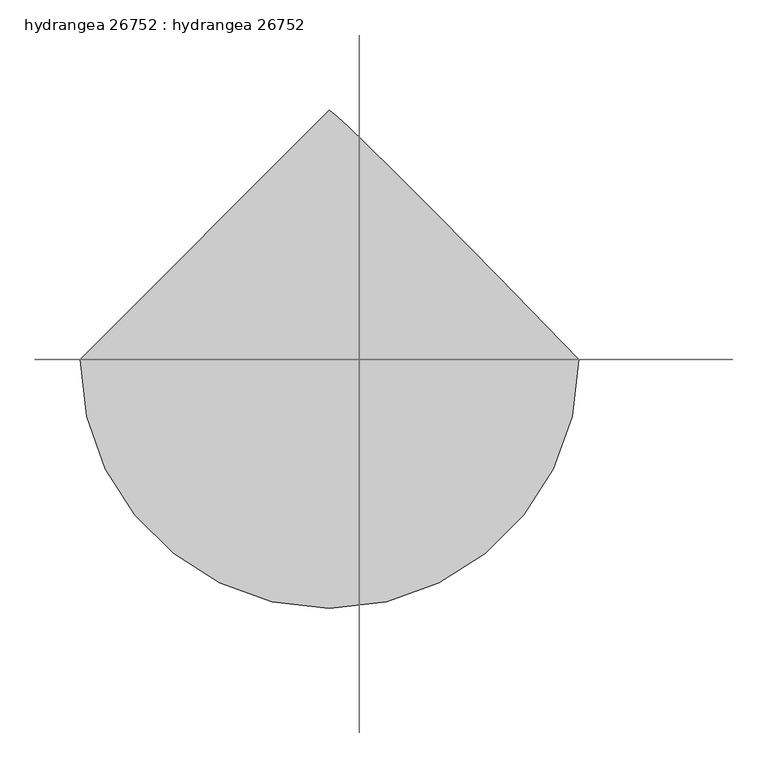
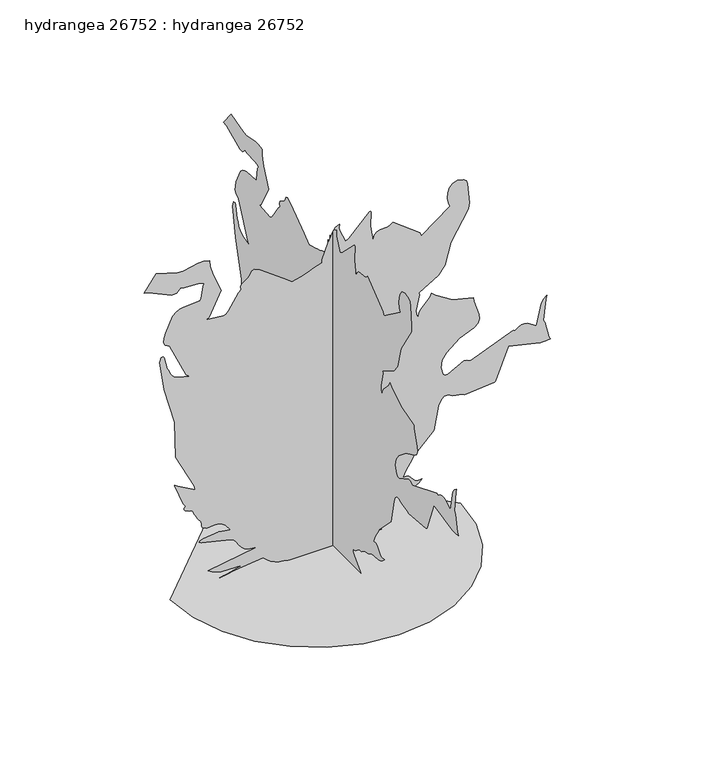
"""IFC4 building model written with IfcOpenShell, lengths in millimetres: proxy geometry, hydrangea 26752 : hydrangea 26752."""

import ifcopenshell
import ifcopenshell.guid

model = None  # the IFC model being written
_history = None  # IfcOwnerHistory: only IFC2X3 demands one
_inside = {}  # id of a spatial element -> (the spatial element, [elements in it])
_under = {}  # id of a project, library or spatial element -> (it, [spatial elements below it])
_declared = {}  # id of a project -> (the project, [libraries it declares])
_typed = {}  # id of a type object -> (the type object, [elements of that type])
_made_of = {}  # id of a material, layer set ... -> (it, [elements and type objects made of it])


def new_model(schema):
    """Start an empty IFC model of exactly this schema.

    Asked for "IFC4X3", IfcOpenShell would pick the latest addendum, in which some entities
    have other attributes; the version numbers below select the first issue.
    IFC2X3 requires an IfcOwnerHistory on every rooted entity: one is made here for all.
    """
    global model, _history
    if schema == "IFC4X3":
        model = ifcopenshell.file(schema_version=(4, 3, 0, 0))
    else:
        model = ifcopenshell.file(schema=schema)
    _inside.clear()
    _under.clear()
    _declared.clear()
    _typed.clear()
    _made_of.clear()
    _history = None
    if model.schema == "IFC2X3":
        org = make("IfcOrganization", Name="unknown")
        user = make(
            "IfcPersonAndOrganization",
            ThePerson=make("IfcPerson", FamilyName="unknown"),
            TheOrganization=org,
        )
        app = make(
            "IfcApplication",
            ApplicationDeveloper=org,
            Version="unknown",
            ApplicationFullName="unknown",
            ApplicationIdentifier="unknown",
        )
        _history = make(
            "IfcOwnerHistory",
            OwningUser=user,
            OwningApplication=app,
            ChangeAction="ADDED",
            CreationDate=0,
        )
    return model


def make(cls, **values):
    """One entity of the class cls with the attributes given. An attribute that is None is left unset."""
    return model.create_entity(
        cls, **{name: value for name, value in values.items() if value is not None}
    )


def rooted(cls, **values):
    """An entity with a GlobalId (a new one), such as an element, a storey or a relation."""
    return make(cls, GlobalId=ifcopenshell.guid.new(), OwnerHistory=_history, **values)


def si_unit(unit_type, name, prefix=None):
    """IfcSIUnit, for example si_unit("LENGTHUNIT", "METRE", prefix="MILLI")."""
    return make("IfcSIUnit", UnitType=unit_type, Prefix=prefix, Name=name)


def assignment(units):
    """IfcUnitAssignment: the units of a project."""
    return None if units is None else make("IfcUnitAssignment", Units=units)


def point(xyz):
    """IfcCartesianPoint."""
    return None if xyz is None else make("IfcCartesianPoint", Coordinates=xyz)


def direction(xyz):
    """IfcDirection."""
    return None if xyz is None else make("IfcDirection", DirectionRatios=xyz)


def frame(location, z_axis=None, x_axis=None):
    """IfcAxis2Placement3D, a coordinate frame: its origin and axes. An axis left out is left unset."""
    return make(
        "IfcAxis2Placement3D",
        Location=point(location),
        Axis=direction(z_axis),
        RefDirection=direction(x_axis),
    )


def origin():
    """The frame at (0, 0, 0) with its axes left unset."""
    return frame((0.0, 0.0, 0.0))


def place(relative_to, where):
    """IfcLocalPlacement: puts the frame where relative to a parent placement (None: the world)."""
    return make(
        "IfcLocalPlacement", PlacementRelTo=relative_to, RelativePlacement=where
    )


def context(
    kind, dimensions, precision=None, world=None, true_north=None, identifier=None
):
    """IfcGeometricRepresentationContext, for example the 3D "Model" context."""
    return make(
        "IfcGeometricRepresentationContext",
        ContextIdentifier=identifier,
        ContextType=kind,
        CoordinateSpaceDimension=dimensions,
        Precision=precision,
        WorldCoordinateSystem=world,
        TrueNorth=true_north,
    )


def project(units=None, contexts=None):
    """IfcProject with its units and contexts."""
    return rooted(
        "IfcProject",
        Name="project",
        RepresentationContexts=contexts,
        UnitsInContext=assignment(units),
    )


def spatial(cls, under=None, at=None, **own):
    """A site, building, storey or space (cls), placed at a placement, below another one or the project."""
    s = rooted(cls, ObjectPlacement=at, **own)
    if under is not None:
        _under.setdefault(under.id(), (under, []))[1].append(s)
    return s


def point_list(points):
    """IfcCartesianPointList2D or 3D."""
    cls = (
        "IfcCartesianPointList2D" if len(points[0]) == 2 else "IfcCartesianPointList3D"
    )
    return make(cls, CoordList=points)


def triangles(points, corners, closed=None, point_numbers=None):
    """IfcTriangulatedFaceSet: each triangle names its three corners, points numbered from 1."""
    return make(
        "IfcTriangulatedFaceSet",
        Coordinates=point_list(points),
        Closed=closed,
        CoordIndex=corners,
        PnIndex=point_numbers,
    )


def shape(context_of_items, identifier, shape_type, items):
    """IfcShapeRepresentation: the items that make up one representation, for example the "Body"."""
    return make(
        "IfcShapeRepresentation",
        ContextOfItems=context_of_items,
        RepresentationIdentifier=identifier,
        RepresentationType=shape_type,
        Items=items,
    )


def source(mapping_origin, context_of_items, identifier, shape_type, items):
    """IfcRepresentationMap: a shape defined once, which mapped items show again and again."""
    return make(
        "IfcRepresentationMap",
        MappingOrigin=mapping_origin,
        MappedRepresentation=shape(context_of_items, identifier, shape_type, items),
    )


def transform(
    local_origin,
    x_axis=None,
    y_axis=None,
    z_axis=None,
    scale=None,
    scale2=None,
    scale3=None,
    uniform=True,
):
    """IfcCartesianTransformationOperator3D, or its non-uniform kind. x_axis, y_axis, z_axis: its Axis1, 2, 3."""
    if uniform:
        return make(
            "IfcCartesianTransformationOperator3D",
            Axis1=direction(x_axis),
            Axis2=direction(y_axis),
            LocalOrigin=point(local_origin),
            Scale=scale,
            Axis3=direction(z_axis),
        )
    return make(
        "IfcCartesianTransformationOperator3DnonUniform",
        Axis1=direction(x_axis),
        Axis2=direction(y_axis),
        LocalOrigin=point(local_origin),
        Scale=scale,
        Axis3=direction(z_axis),
        Scale2=scale2,
        Scale3=scale3,
    )


def mapped(mapping_source, mapping_target):
    """IfcMappedItem: shows the shape of a source again, moved by a transform."""
    return make(
        "IfcMappedItem", MappingSource=mapping_source, MappingTarget=mapping_target
    )


def made_of(thing, what):
    """Note that an element or type object is made of a material, layer set ...; save() writes the relation."""
    if what is not None:
        _made_of.setdefault(what.id(), (what, []))[1].append(thing)
    return thing


def element(
    cls,
    number,
    at=None,
    inside=None,
    cuts=None,
    type_object=None,
    material=None,
    context=None,
    identifier="Body",
    shape_type=None,
    held_by="IfcProductDefinitionShape",
    body=None,
    shapes=None,
    **own,
):
    """One element of the class cls, such as IfcWall. Its Tag is "e" and its number.

    at: its placement. inside: the storey or other place that contains it. cuts: it is an
    opening in that element (IfcRelVoidsElement). A single representation is given by context,
    identifier, shape_type and body (its items); several are given by shapes. held_by: the class
    of the entity that holds the representations. save() writes the other relations.
    """
    e = rooted(cls, Tag="e%d" % number, ObjectPlacement=at, **own)
    if body is not None:
        shapes = [shape(context, identifier, shape_type, body)]
    if shapes is not None:
        e.Representation = make(held_by, Representations=shapes)
    if inside is not None:
        _inside.setdefault(inside.id(), (inside, []))[1].append(e)
    if cuts is not None:
        rooted(
            "IfcRelVoidsElement", RelatingBuildingElement=cuts, RelatedOpeningElement=e
        )
    if type_object is not None:
        _typed.setdefault(type_object.id(), (type_object, []))[1].append(e)
    return made_of(e, material)


def aggregate(whole, parts):
    """IfcRelAggregates: a whole, such as a stair, and the parts it consists of."""
    return rooted("IfcRelAggregates", RelatingObject=whole, RelatedObjects=parts)


def save(model, path):
    """Write the relations noted so far, then the file.

    IfcRelAggregates (storeys below a building ...), IfcRelContainedInSpatialStructure (elements
    in a storey), IfcRelDefinesByType, IfcRelAssociatesMaterial and IfcRelDeclares: one each for
    every whole, place, type object, material and project.
    """
    for whole, parts in _under.values():
        aggregate(whole, parts)
    for where, things in _inside.values():
        rooted(
            "IfcRelContainedInSpatialStructure",
            RelatedElements=things,
            RelatingStructure=where,
        )
    for kind, things in _typed.values():
        rooted("IfcRelDefinesByType", RelatedObjects=things, RelatingType=kind)
    for what, things in _made_of.values():
        rooted("IfcRelAssociatesMaterial", RelatedObjects=things, RelatingMaterial=what)
    for by, libraries in _declared.values():
        rooted("IfcRelDeclares", RelatingContext=by, RelatedDefinitions=libraries)
    model.write(path)


def hydrangea_26752_hydrangea_26752_6cd4de68(model_context):
    return source(origin(), model_context, "Body", "Tessellation", [
        triangles([(-464.7672343, 0.0, 3.02e-05), (-452.4787039, -106.4936905, 3.02e-05), (-417.4875984, -204.2914365, 3.02e-05), (-362.5905132, -290.5916013, 3.02e-05), (-290.5916013, -362.5905132, 3.02e-05), (-204.2911822, -417.4875984, 3.02e-05), (-106.4936905, -452.4787039, 3.02e-05), (2.03e-05, -464.7672343, 3.02e-05), (106.4939449, -452.4787039, 3.02e-05), (204.2914365, -417.4875984, 3.02e-05), (290.5916013, -362.5905132, 3.02e-05), (362.5905132, -290.5916013, 3.02e-05), (417.4875984, -204.2911822, 3.02e-05), (452.4787039, -106.4936905, 3.02e-05), (464.7672343, 4.06e-05, 3.02e-05), (313.7284884, 154.9290062, 3.02e-05), (201.7549816, 268.9964805, 3.02e-05), (122.337727, 349.0116546, 3.02e-05), (68.9646404, 401.7878663, 3.02e-05), (35.1246865, 434.1297149, 3.02e-05), (14.3067201, 452.8546257, 3.02e-05), (-6.09e-05, 464.7672343, 3.02e-05), (56.0289111, -377.7746518, 894.66276), (56.0289111, -434.8662978, 988.0256659), (56.0289111, -437.025323, 1007.8783058), (56.0289111, -431.6938534, 1074.0784075), (56.0289111, -427.5688871, 1084.5381615), (56.0289111, -420.2181004, 1091.4545998), (56.0289111, -399.2732306, 1096.0341894), (56.0289111, -384.089092, 1091.3859993), (56.0289111, -374.1170626, 1079.9991943), (56.0289111, -368.8109911, 1064.3553091), (56.0289111, -367.6197121, 1046.9435812), (56.0289111, -369.9971832, 1030.2455452), (56.0289111, -375.3946735, 1016.7479679), (56.0289111, -283.8809099, 949.5141357), (56.0289111, -278.4503729, 960.8348837), (56.0289111, -192.0161139, 1027.487138), (56.0289111, -183.512436, 1019.3997683), (56.0289111, -173.3158381, 1016.575304), (56.0289111, -151.4921339, 1016.077442), (56.0289111, -141.6905156, 1013.0776978), (56.0289111, -133.8441922, 1004.6956512), (56.0289111, -128.8665527, 988.2669302), (56.0289111, -120.2805761, 1038.0128763), (56.0289111, -121.9587531, 1087.6699471), (56.0289111, -121.3283319, 1088.8815737), (56.0289111, -120.3204537, 1089.2625824), (56.0289111, -119.0941387, 1088.975536), (56.0289111, -117.8101691, 1088.1856133), (56.0289111, -51.0174846, 1022.5290831), (56.0289111, -40.1538944, 1015.3484894), (56.0289111, -21.3923125, 1059.6105406), (56.0289111, -19.9031842, 1068.9729778), (56.0289111, -20.5441289, 1080.248089), (56.0289111, -9.1964113, 1074.4568727), (56.0289111, -0.5405762, 1063.7304199), (56.0289111, 13.2029357, 1031.7950146), (56.0289111, 15.0194446, 1031.1828426), (56.0289111, 16.1084712, 1040.5605406), (56.0289111, 15.8290449, 1030.10333), (56.0289111, 34.9326629, 980.1719301), (56.0289111, 34.6535171, 969.7147923), (56.0289111, 46.9016657, 965.6583538), (56.0289111, 59.853396, 960.979715), (56.0289111, 73.3885619, 956.0013124), (56.0289111, 87.3888065, 951.0482718), (56.0289111, 101.7342336, 946.4457911), (56.0289111, 116.3062366, 942.5138363), (56.0289111, 130.9854187, 939.5776056), (56.0289111, 158.8299491, 961.2921232), (56.0289111, 234.3038488, 1015.5618484), (56.0289111, 252.5433605, 1023.7431805), (56.0289111, 260.6957517, 1020.4259411), (56.0289111, 264.4829115, 1008.7952557), (56.0289111, 270.9573709, 1001.4368385), (56.0289111, 292.1841821, 987.7081707), (56.0289111, 295.084859, 980.1414814), (56.0289111, 293.5100641, 968.1907574), (56.0289111, 301.5567932, 960.9593674), (56.0289111, 333.5786213, 911.8103325), (56.0289111, 341.9555446, 903.575588), (56.0289111, 350.6474195, 900.6063652), (56.0289111, 405.2778059, 906.5576008), (56.0289111, 397.091387, 912.3182957), (56.0289111, 357.3022459, 989.5521715), (56.0289111, 383.3829941, 1051.2462982), (56.0289111, 392.869915, 1083.2706516), (56.0289111, 394.0713315, 1102.6610378), (56.0289111, 413.8020676, 1107.4693199), (56.0289111, 431.2518745, 1106.8977705), (56.0289111, 479.0928497, 1096.097703), (56.0289111, 496.5959965, 1097.2025774), (56.0289111, 565.8923844, 1117.6013323), (56.0289111, 605.1150993, 1065.3077946), (56.0289111, 590.4389603, 1063.2046526), (56.0289111, 515.963528, 1028.2542423), (56.0289111, 499.8980115, 1030.0398165), (56.0289111, 487.4520052, 1042.8973166), (56.0289111, 476.9008324, 1039.305748), (56.0289111, 431.2823596, 1037.8351255), (56.0289111, 421.2823886, 1035.6633831), (56.0289111, 412.7479531, 1030.7561245), (56.0289111, 416.4106656, 1023.8879391), (56.0289111, 422.1561361, 984.398489), (56.0289111, 425.8213557, 977.5278328), (56.0289111, 478.1860737, 974.7465345), (56.0289111, 490.5939646, 971.7493338), (56.0289111, 502.2144762, 965.7473019), (56.0289111, 512.7834532, 955.7015488), (56.0289111, 536.4029417, 906.3493286), (56.0289111, 540.7590348, 890.4260273), (56.0289111, 541.4473649, 876.4001392), (56.0289111, 536.9465132, 865.9378418), (56.0289111, 523.4413055, 857.3729576), (56.0289111, 470.3247439, 742.9737631), (56.0289111, 459.1462111, 734.3275612), (56.0289111, 495.4784048, 743.0092987), (56.0289111, 506.2683349, 747.8099504), (56.0289111, 515.3336246, 754.7263887), (56.0289111, 522.0366674, 764.454574), (56.0289111, 525.7400024, 777.6930828), (56.0289111, 531.1476665, 784.7339321), (56.0289111, 539.8243172, 825.0565435), (56.0289111, 543.8298866, 829.879941), (56.0289111, 550.6015663, 829.2856459), (56.0289111, 555.6434461, 813.3064613), (56.0289111, 540.8123746, 716.5628025), (56.0289111, 507.4392663, 594.6655191), (56.0289111, 503.093347, 475.8365441), (56.0289111, 444.0484045, 359.0446904), (56.0289111, 441.1045435, 344.0002235), (56.0289111, 497.2995872, 374.7622267), (56.0289111, 506.1286268, 381.752316), (56.0289111, 507.3122755, 379.8777938), (56.0289111, 479.3442879, 309.3622215), (56.0289111, 471.5769931, 298.1760402), (56.0289111, 476.8474926, 293.4109968), (56.0289111, 476.8347754, 288.7729441), (56.0289111, 473.0577893, 284.5159002), (56.0289111, 460.289201, 278.1963731), (56.0289111, 454.3303714, 276.6495199), (56.0289111, 450.6829196, 276.5250544), (56.0289111, 447.9727289, 270.8405358), (56.0289111, 445.4428688, 265.374445), (56.0289111, 442.9105016, 259.9769365), (56.0289111, 440.1901734, 254.4981467), (56.0289111, 437.1015175, 248.789756), (56.0289111, 433.4642395, 242.6990667), (56.0289111, 429.0903422, 236.0780501), (56.0289111, 423.9341526, 231.4173971), (56.0289111, 421.2519035, 226.5421133), (56.0289111, 420.2282742, 221.6594716), (56.0289111, 420.0530305, 216.9764544), (56.0289111, 419.910779, 212.7001166), (56.0289111, 418.9912857, 209.0374223), (56.0289111, 416.4817732, 206.1956808), (56.0289111, 404.3481751, 201.1304013), (56.0289111, 392.979138, 200.8065475), (56.0289111, 381.7802576, 202.325223), (56.0289111, 370.1622894, 202.7872406), (56.0289111, 357.5257424, 199.293722), (56.0289111, 343.2814084, 188.9454982), (56.0289111, 326.8374267, 168.843146), (56.0289111, 363.7335394, 174.8182537), (56.0289111, 415.2447847, 168.959745), (56.0289111, 424.7621907, 165.1799612), (56.0289111, 427.6882476, 161.3724901), (56.0289111, 422.6031655, 158.3819023), (56.0289111, 326.8374267, 135.2257031), (56.0289111, 316.3675352, 128.5444794), (56.0289111, 308.4071926, 119.1548454), (56.0289111, 301.2011826, 108.4708318), (56.0289111, 292.9842786, 97.9059425), (56.0289111, 281.9936886, 88.8741991), (56.0289111, 266.4742689, 82.7891145), (56.0289111, 244.6604659, 81.0642016), (56.0289111, 399.6745505, 54.9174055), (56.0289111, 387.1320385, 46.4490362), (56.0289111, 358.6535079, 37.4287247), (56.0289111, 291.3510571, 36.2410178), (56.0289111, 337.9144032, 23.9287606), (56.0289111, 349.4180614, 21.3156048), (56.0289111, 362.3212709, 18.4984871), (56.0289111, 355.630909, 19.454849), (56.0289111, 338.5316257, 22.4599004), (56.0289111, 314.6454383, 26.6484415), (56.0289111, 223.7308386, 37.9362155), (56.0289111, 211.5466986, 26.1533955), (56.0289111, 198.7755668, 17.3074794), (56.0289111, 185.515475, 10.9090339), (56.0289111, 171.8642371, 6.4684733), (56.0289111, 157.9193579, 3.4965937), (56.0289111, 143.7791599, 1.5035523), (56.0289111, 129.5409211, 0.0), (56.0289111, -156.3006158, 8.5e-06), (56.0289111, -151.6640893, 6.8894283), (56.0289111, -116.3057279, 38.9204668), (56.0289111, -111.4957199, 47.331436), (56.0289111, -111.590972, 55.6176853), (56.0289111, -119.3379828, 56.8782915), (56.0289111, -125.2241879, 59.5351333), (56.0289111, -130.2038621, 63.1188217), (56.0289111, -135.2315439, 67.1597133), (56.0289111, -141.2622714, 71.1881602), (56.0289111, -149.2498198, 74.7345099), (56.0289111, -160.1494906, 77.329128), (56.0289111, -168.9650681, 83.9521794), (56.0289111, -176.5355544, 87.5539036), (56.0289111, -196.7577757, 92.3169214), (56.0289111, -204.3280077, 95.9186456), (56.0289111, -213.1436033, 102.5419604), (56.0289111, -254.4092531, 106.5686224), (56.0289111, -265.3388912, 110.053257), (56.0289111, -275.7884532, 116.2788036), (56.0289111, -285.3972962, 126.1210626), (56.0289111, -270.7287694, 125.7187253), (56.0289111, -261.0386631, 129.5500684), (56.0289111, -244.0602664, 149.2523633), (56.0289111, -236.5088377, 152.8248832), (56.0289111, -225.0498715, 152.0344246), (56.0289111, -234.5898597, 172.6625532), (56.0289111, -246.2180017, 193.2690897), (56.0289111, -259.5756166, 213.3033683), (56.0289111, -323.1010995, 276.6977727), (56.0289111, -338.0566183, 354.6326777), (56.0289111, -345.6055398, 371.0131823), (56.0289111, -356.2354506, 380.7922002), (56.0289111, -370.7261358, 381.2874825), (56.0289111, -376.1719153, 376.5935466), (56.0289111, -382.951189, 373.9163844), (56.0289111, -414.431971, 368.0820022), (56.0289111, -421.1503109, 364.0103757), (56.0289111, -516.6848866, 372.087608), (56.0289111, -521.0689213, 374.2821688), (56.0289111, -561.6327971, 477.6729873), (56.0289111, -663.3141632, 454.759633), (56.0289111, -683.0017696, 454.2617709), (56.0289111, -696.6263014, 456.4588752), (56.0289111, -691.4650612, 464.9628256), (56.0289111, -679.3771362, 518.9251568), (56.0289111, -674.215896, 527.4291072), (56.0289111, -681.6479279, 594.9220805), (56.0289111, -685.4224068, 606.8042041), (56.0289111, -674.9575659, 597.7338638), (56.0289111, -667.4314991, 587.1039531), (56.0289111, -651.805418, 516.2225965), (56.0289111, -623.5224787, 533.9975653), (56.0289111, -613.96703, 536.3114865), (56.0289111, -604.0863831, 535.7831758), (56.0289111, -593.7181206, 531.7852003), (56.0289111, -582.7021142, 523.6927437), (56.0289111, -577.4646432, 527.2970295), (56.0289111, -440.4085831, 471.9960809), (56.0289111, -429.7609045, 477.805065), (56.0289111, -420.0225454, 479.0471403), (56.0289111, -367.9321567, 451.6074635), (56.0289111, -358.5290606, 450.3882792), (56.0289111, -353.3322121, 456.9262522), (56.0289111, -345.7960078, 481.3356634), (56.0289111, -350.0683125, 504.1753667), (56.0289111, -363.3880663, 525.0059266), (56.0289111, -406.1337856, 558.9200629), (56.0289111, -451.9579871, 579.6160017), (56.0289111, -465.1685543, 589.0190978), (56.0289111, -469.6389573, 603.0043633), (56.0289111, -467.9142806, 619.826774), (56.0289111, -451.0918336, 669.8597666), (56.0289111, -450.0987256, 680.5760456), (56.0289111, -383.0096157, 698.4017744), (56.0289111, -329.3240845, 731.7240864), (56.0289111, -316.5631265, 743.6087534), (56.0289111, -311.5136164, 731.6199503), (56.0289111, -280.6932047, 700.0375757), (56.0289111, -275.2499687, 690.0807707), (56.0289111, -272.6744173, 676.8397184), (56.0289111, -266.9721128, 689.0418806), (56.0289111, -265.8748323, 702.5623489), (56.0289111, -277.0838502, 752.2879475), (56.0289111, -276.1770741, 759.2500952), (56.0289111, -338.0413939, 796.367161), (56.0289111, -358.8363819, 823.4360029), (433.8020459, 5.25e-05, 894.66276), (490.8936919, 6.21e-05, 988.0256659), (493.0552242, 6.39e-05, 1007.8783058), (487.7237909, 6.93e-05, 1074.0784075), (483.5988247, 7.01e-05, 1084.5381615), (476.2454945, 7.04e-05, 1091.4545998), (455.3006247, 7.02e-05, 1096.0341894), (440.1164861, 6.93e-05, 1091.3859993), (430.1470001, 6.81e-05, 1079.9991943), (424.8383852, 6.66e-05, 1064.3553091), (423.6496496, 6.51e-05, 1046.9435812), (426.0270844, 6.37e-05, 1030.2455452), (431.4246111, 6.27e-05, 1016.7479679), (339.9082858, 5.44e-05, 949.5141357), (334.477767, 5.52e-05, 960.8348837), (248.0447615, 5.82e-05, 1027.487138), (239.541338, 5.73e-05, 1019.3997683), (229.3447583, 5.67e-05, 1016.575304), (207.5210541, 5.6e-05, 1016.077442), (197.7191814, 5.55e-05, 1013.0776978), (189.8731124, 5.45e-05, 1004.6956512), (184.8952004, 5.3e-05, 988.2669302), (176.3092419, 5.66e-05, 1038.0128763), (177.9874098, 6.11e-05, 1087.6699471), (177.3572339, 6.11e-05, 1088.8815737), (176.3491196, 6.1e-05, 1089.2625824), (175.1227954, 6.09e-05, 1088.975536), (173.8390802, 6.07e-05, 1088.1856133), (107.0464002, 5.35e-05, 1022.5290831), (96.182801, 5.27e-05, 1015.3484894), (77.4210737, 5.59e-05, 1059.6105406), (75.9321248, 5.66e-05, 1068.9729778), (76.5729696, 5.75e-05, 1080.248089), (65.2252475, 5.67e-05, 1074.4568727), (56.5694259, 5.55e-05, 1063.7304199), (42.8259742, 5.23e-05, 1031.7950146), (41.0093655, 5.23e-05, 1031.1828426), (39.9204648, 5.31e-05, 1040.5605406), (40.1998673, 5.22e-05, 1030.10333), (21.0960983, 4.75e-05, 980.1719301), (21.3753963, 4.66e-05, 969.7147923), (9.1270438, 4.59e-05, 965.6583538), (-3.8244574, 4.51e-05, 960.979715), (-17.3597019, 4.43e-05, 956.0013124), (-31.3598954, 4.34e-05, 951.0482718), (-45.7053225, 4.26e-05, 946.4457911), (-60.2773209, 4.18e-05, 942.5138363), (-74.9565076, 4.11e-05, 939.5776056), (-102.801038, 4.21e-05, 961.2921232), (-178.2749468, 4.45e-05, 1015.5618484), (-196.5144585, 4.46e-05, 1023.7431805), (-204.6668497, 4.41e-05, 1020.4259411), (-208.4534826, 4.3e-05, 1008.7952557), (-214.9284508, 4.22e-05, 1001.4368385), (-236.1547533, 4.05e-05, 987.7081707), (-239.055957, 3.97e-05, 980.1414814), (-237.481907, 3.88e-05, 968.1907574), (-245.5273643, 3.79e-05, 960.9593674), (-277.5486837, 3.28e-05, 911.8103325), (-285.9281505, 3.19e-05, 903.575588), (-294.6200436, 3.14e-05, 900.6063652), (-349.2479047, 3.02e-05, 906.5576008), (-341.0639929, 3.09e-05, 912.3182957), (-301.2723083, 3.86e-05, 989.5521715), (-327.3530565, 4.31e-05, 1051.2462982), (-336.8399775, 4.55e-05, 1083.2706516), (-338.0413939, 4.71e-05, 1102.6610378), (-357.77213, 4.69e-05, 1107.4693199), (-375.2244804, 4.63e-05, 1106.8977705), (-423.0654556, 4.4e-05, 1096.097703), (-440.5660953, 4.36e-05, 1097.2025774), (-509.8649903, 4.32e-05, 1117.6013323), (-549.0851618, 3.76e-05, 1065.3077946), (-534.4115662, 3.79e-05, 1063.2046526), (-459.9361339, 3.72e-05, 1028.2542423), (-443.8706174, 3.78e-05, 1030.0398165), (-431.4246111, 3.93e-05, 1042.8973166), (-420.8734383, 3.93e-05, 1039.305748), (-375.252422, 4.05e-05, 1037.8351255), (-365.252451, 4.06e-05, 1035.6633831), (-356.7180519, 4.05e-05, 1030.7561245), (-360.3832715, 3.98e-05, 1023.8879391), (-366.128742, 3.63e-05, 984.398489), (-369.7914182, 3.56e-05, 977.5278328), (-422.1586796, 3.38e-05, 974.7465345), (-434.5666068, 3.32e-05, 971.7493338), (-446.184575, 3.23e-05, 965.7473019), (-456.7535156, 3.12e-05, 955.7015488), (-480.3730042, 2.63e-05, 906.3493286), (-484.7290973, 2.48e-05, 890.4260273), (-485.4174637, 2.36e-05, 876.4001392), (-480.9165756, 2.29e-05, 865.9378418), (-467.4139114, 2.25e-05, 857.3729576), (-414.2948427, 1.45e-05, 742.9737631), (-403.118817, 1.41e-05, 734.3275612), (-439.4484673, 1.37e-05, 743.0092987), (-450.2383973, 1.38e-05, 747.8099504), (-459.303687, 1.42e-05, 754.7263887), (-466.0067662, 1.48e-05, 764.454574), (-469.7100649, 1.58e-05, 777.6930828), (-475.117729, 1.62e-05, 784.7339321), (-483.7943796, 1.93e-05, 825.0565435), (-487.7999854, 1.96e-05, 829.879941), (-494.5741722, 1.93e-05, 829.2856459), (-499.6160883, 1.78e-05, 813.3064613), (-484.782437, 1.01e-05, 716.5628025), (-451.4119085, 9e-07, 594.6655191), (-447.0659529, -9e-06, 475.8365441), (-388.0210467, -1.71e-05, 359.0446904), (-385.0746423, -1.83e-05, 344.0002235), (-441.2721931, -1.73e-05, 374.7622267), (-450.1012327, -1.7e-05, 381.752316), (-451.2848814, -1.73e-05, 379.8777938), (-423.3143867, -2.24e-05, 309.3622215), (-415.549599, -2.3e-05, 298.1760402), (-420.817555, -2.36e-05, 293.4109968), (-420.8048378, -2.39e-05, 288.7729441), (-417.0303952, -2.41e-05, 284.5159002), (-404.2592634, -2.42e-05, 278.1963731), (-398.3029773, -2.42e-05, 276.6495199), (-394.6555255, -2.42e-05, 276.5250544), (-391.9453348, -2.46e-05, 270.8405358), (-389.4129676, -2.5e-05, 265.374445), (-386.880564, -2.54e-05, 259.9769365), (-384.1602359, -2.58e-05, 254.4981467), (-381.0741234, -2.62e-05, 248.789756), (-377.4343019, -2.65e-05, 242.6990667), (-373.0604047, -2.7e-05, 236.0780501), (-367.9067585, -2.72e-05, 231.4173971), (-365.221966, -2.76e-05, 226.5421133), (-364.1983366, -2.8e-05, 221.6594716), (-364.0230929, -2.84e-05, 216.9764544), (-363.8808414, -2.87e-05, 212.7001166), (-362.9613482, -2.9e-05, 209.0374223), (-360.4543791, -2.92e-05, 206.1956808), (-348.320781, -2.92e-05, 201.1304013), (-336.9492004, -2.89e-05, 200.8065475), (-325.7528635, -2.84e-05, 202.325223), (-314.1323519, -2.81e-05, 202.7872406), (-301.4983665, -2.8e-05, 199.293722), (-287.2540325, -2.84e-05, 188.9454982), (-270.8075073, -2.96e-05, 168.843146), (-307.7036018, -3e-05, 174.8182537), (-359.2173906, -3.17e-05, 168.959745), (-368.7322532, -3.24e-05, 165.1799612), (-371.6583464, -3.32e-05, 161.3724901), (-366.5732643, -3.31e-05, 158.3819023), (-270.8075073, -3.24e-05, 135.2257031), (-260.3376158, -3.27e-05, 128.5444794), (-252.3792717, -3.32e-05, 119.1548454), (-245.1717719, -3.39e-05, 108.4708318), (-236.9543411, -3.46e-05, 97.9059425), (-225.9652771, -3.51e-05, 88.8741991), (-210.44484, -3.51e-05, 82.7891145), (-188.6315457, -3.46e-05, 81.0642016), (-343.6446493, -4.14e-05, 54.9174055), (-331.1021009, -4.15e-05, 46.4490362), (-302.6235885, -4.14e-05, 37.4287247), (-235.3221369, -3.98e-05, 36.2410178), (-281.887009, -4.21e-05, 23.9287856), (-293.3906855, -4.27e-05, 21.3156298), (-306.2913697, -4.33e-05, 18.498512), (-299.6009896, -4.31e-05, 19.454874), (-282.5016881, -4.23e-05, 22.4599277), (-258.6180442, -4.13e-05, 26.6484415), (-167.7021728, -3.76e-05, 37.9362155), (-155.5177784, -3.82e-05, 26.1533955), (-142.7466466, -3.86e-05, 17.3074794), (-129.4865639, -3.88e-05, 10.9090589), (-115.8353169, -3.87e-05, 6.4684733), (-101.8904468, -3.85e-05, 3.496619), (-87.7502488, -3.83e-05, 1.5035625), (-73.5122598, -3.8e-05, 9.2e-06), (212.3292817, -2.95e-05, 5.3e-06), (207.6930094, -2.9e-05, 6.8894283), (172.3346299, -2.74e-05, 38.9204668), (167.52464, -2.68e-05, 47.331436), (167.6196379, -2.61e-05, 55.6176853), (175.3668939, -2.58e-05, 56.8782915), (181.2528355, -2.54e-05, 59.5351333), (186.2325279, -2.49e-05, 63.1188217), (191.2602007, -2.44e-05, 67.1597133), (197.2911916, -2.39e-05, 71.1881602), (205.2787309, -2.34e-05, 74.7345099), (216.1781383, -2.29e-05, 77.329128), (224.9937339, -2.2e-05, 83.9521794), (232.5642021, -2.15e-05, 87.5539036), (252.7864416, -2.05e-05, 92.3169214), (260.3579453, -2e-05, 95.9186456), (269.1717423, -1.91e-05, 102.5419604), (310.4366472, -1.75e-05, 106.5686224), (321.3688288, -1.69e-05, 110.0530027), (331.8183726, -1.61e-05, 116.2788036), (341.4272338, -1.5e-05, 126.1210626), (326.7586887, -1.55e-05, 125.7187253), (317.0660391, -1.54e-05, 129.5500684), (300.0886597, -1.43e-05, 149.2523633), (292.5372311, -1.42e-05, 152.8248832), (281.0792822, -1.46e-05, 152.0344246), (290.6195429, -1.26e-05, 172.6625532), (302.2476667, -1.05e-05, 193.2690897), (315.6030107, -8.4e-06, 213.3033683), (379.1284936, -1.2e-06, 276.6977727), (394.0840124, 5.8e-06, 354.6326777), (401.6328976, 7.5e-06, 371.0131823), (412.2628083, 8.6e-06, 380.7922002), (426.7535299, 9.1e-06, 381.2874825), (432.1993094, 8.8e-06, 376.5935466), (438.9785831, 8.8e-06, 373.9163844), (470.4619085, 9.3e-06, 368.0820022), (477.1802121, 9.1e-06, 364.0103757), (572.7148241, 1.25e-05, 372.087608), (577.0988588, 1.3e-05, 374.2821688), (617.6601912, 2.29e-05, 477.6729873), (719.3415573, 2.4e-05, 454.759633), (739.0291637, 2.45e-05, 454.2617709), (752.6562389, 2.51e-05, 456.4588752), (747.4949987, 2.57e-05, 464.9628256), (735.4070738, 2.99e-05, 518.9251568), (730.2458336, 3.04e-05, 527.4291072), (737.6778654, 3.63e-05, 594.9220805), (741.4498009, 3.74e-05, 606.8042041), (730.9875034, 3.64e-05, 597.7338638), (723.4614367, 3.53e-05, 587.1039531), (707.8328121, 2.88e-05, 516.2225965), (679.5498728, 2.95e-05, 533.9975653), (669.9969675, 2.94e-05, 536.3114865), (660.1163206, 2.91e-05, 535.7831758), (649.7455147, 2.84e-05, 531.7852003), (638.729472, 2.74e-05, 523.6927437), (633.492001, 2.76e-05, 527.2970295), (496.4359772, 1.88e-05, 471.9960809), (485.7882986, 1.9e-05, 477.805065), (476.0524467, 1.88e-05, 479.0471403), (423.9620942, 1.49e-05, 451.6074635), (414.5564547, 1.45e-05, 450.3882792), (409.3621496, 1.49e-05, 456.9262522), (401.8259454, 1.72e-05, 481.3356634), (406.09825, 1.94e-05, 504.1753667), (419.4180038, 2.15e-05, 525.0059266), (462.1637232, 2.53e-05, 558.9200629), (507.9853812, 2.82e-05, 579.6160017), (521.1984919, 2.94e-05, 589.0190978), (525.6663514, 3.07e-05, 603.0043633), (523.9442182, 3.21e-05, 619.826774), (507.1192277, 3.58e-05, 669.8597666), (506.1286268, 3.66e-05, 680.5760456), (439.0370098, 3.62e-05, 698.4017744), (385.3514786, 3.74e-05, 731.7240864), (372.593064, 3.8e-05, 743.6087534), (367.5409741, 3.68e-05, 731.6199503), (336.7231241, 3.32e-05, 700.0375757), (331.2773809, 3.22e-05, 690.0807707), (328.7043549, 3.11e-05, 676.8397184), (323.0020503, 3.19e-05, 689.0418806), (321.9022264, 3.3e-05, 702.5623489), (333.1112443, 3.76e-05, 752.2879475), (332.2044683, 3.81e-05, 759.2500952), (394.0713315, 4.31e-05, 796.367161), (414.8663195, 4.6e-05, 823.4360029)], [[21, 22, 1], [20, 21, 1], [19, 20, 1], [18, 19, 1], [17, 18, 1], [17, 1, 2], [17, 2, 3], [17, 3, 4], [16, 17, 4], [16, 4, 5], [16, 5, 6], [16, 6, 7], [16, 7, 8], [16, 8, 9], [16, 9, 10], [16, 10, 11], [16, 11, 12], [15, 16, 12], [14, 15, 12], [13, 14, 12], [183, 184, 185], [59, 60, 61], [183, 185, 186], [182, 183, 186], [243, 244, 245], [177, 178, 179], [215, 216, 217], [195, 196, 197], [195, 197, 198], [182, 186, 187], [181, 182, 187], [181, 187, 188], [54, 55, 56], [94, 95, 96], [238, 239, 240], [195, 198, 199], [271, 272, 273], [167, 168, 169], [133, 134, 135], [214, 215, 217], [214, 217, 218], [177, 179, 180], [177, 180, 181], [166, 167, 169], [165, 166, 169], [164, 165, 169], [164, 169, 170], [37, 38, 39], [213, 214, 218], [94, 96, 97], [93, 94, 97], [93, 97, 98], [93, 98, 99], [92, 93, 99], [92, 99, 100], [92, 100, 101], [91, 92, 101], [90, 91, 101], [90, 101, 102], [89, 90, 102], [88, 89, 102], [87, 88, 102], [87, 102, 103], [195, 199, 200], [54, 56, 57], [53, 54, 57], [243, 245, 246], [242, 243, 246], [242, 246, 247], [241, 242, 247], [268, 269, 270], [87, 103, 104], [86, 87, 104], [86, 104, 105], [86, 105, 106], [85, 86, 106], [84, 85, 106], [133, 135, 136], [132, 133, 136], [132, 136, 137], [53, 57, 58], [125, 126, 127], [124, 125, 127], [123, 124, 127], [123, 127, 128], [122, 123, 128], [121, 122, 128], [120, 121, 128], [119, 120, 128], [52, 53, 58], [177, 181, 188], [118, 119, 128], [213, 218, 219], [213, 219, 220], [213, 220, 221], [212, 213, 221], [117, 118, 128], [164, 170, 171], [237, 238, 240], [237, 240, 241], [237, 241, 247], [237, 247, 248], [237, 248, 249], [237, 249, 250], [237, 250, 251], [237, 251, 252], [236, 237, 252], [236, 252, 253], [236, 253, 254], [235, 236, 254], [234, 235, 254], [233, 234, 254], [232, 233, 254], [232, 254, 255], [232, 255, 256], [232, 256, 257], [231, 232, 257], [230, 231, 257], [229, 230, 257], [229, 257, 258], [228, 229, 258], [84, 106, 107], [84, 107, 108], [84, 108, 109], [84, 109, 110], [84, 110, 111], [84, 111, 112], [84, 112, 113], [84, 113, 114], [84, 114, 115], [84, 115, 116], [84, 116, 117], [83, 84, 117], [270, 271, 273], [73, 74, 75], [72, 73, 75], [137, 138, 139], [137, 139, 140], [137, 140, 141], [132, 137, 141], [132, 141, 142], [132, 142, 143], [72, 75, 76], [227, 228, 258], [227, 258, 259], [117, 128, 129], [224, 225, 226], [46, 47, 48], [46, 48, 49], [46, 49, 50], [45, 46, 50], [45, 50, 51], [44, 45, 51], [44, 51, 52], [211, 212, 221], [210, 211, 221], [209, 210, 221], [82, 83, 117], [270, 273, 274], [270, 274, 275], [270, 275, 276], [264, 265, 266], [264, 266, 267], [264, 267, 268], [264, 268, 270], [263, 264, 270], [263, 270, 276], [262, 263, 276], [261, 262, 276], [52, 58, 59], [52, 59, 61], [52, 61, 62], [52, 62, 63], [44, 52, 63], [260, 261, 276], [71, 72, 76], [71, 76, 77], [71, 77, 78], [71, 78, 79], [71, 79, 80], [70, 71, 80], [70, 80, 81], [70, 81, 82], [70, 82, 117], [70, 117, 129], [70, 129, 130], [70, 130, 131], [69, 70, 131], [68, 69, 131], [67, 68, 131], [67, 131, 132], [66, 67, 132], [65, 66, 132], [64, 65, 132], [63, 64, 132], [44, 63, 132], [132, 143, 144], [44, 132, 144], [44, 144, 145], [44, 145, 146], [44, 146, 147], [44, 147, 148], [44, 148, 149], [44, 149, 150], [44, 150, 151], [44, 151, 152], [44, 152, 153], [44, 153, 154], [44, 154, 155], [44, 155, 156], [44, 156, 157], [44, 157, 158], [44, 158, 159], [44, 159, 160], [44, 160, 161], [44, 161, 162], [44, 162, 163], [44, 163, 164], [44, 164, 171], [44, 171, 172], [44, 172, 173], [44, 173, 174], [44, 174, 175], [44, 175, 176], [44, 176, 177], [44, 177, 188], [44, 188, 189], [44, 189, 190], [44, 190, 191], [44, 191, 192], [44, 192, 193], [44, 193, 194], [44, 194, 195], [44, 195, 200], [44, 200, 201], [44, 201, 202], [44, 202, 203], [44, 203, 204], [44, 204, 205], [44, 205, 206], [44, 206, 207], [44, 207, 208], [44, 208, 209], [44, 209, 221], [44, 221, 222], [44, 222, 223], [44, 223, 224], [44, 224, 226], [44, 226, 227], [44, 227, 259], [44, 259, 260], [43, 44, 260], [42, 43, 260], [29, 30, 31], [28, 29, 31], [28, 31, 32], [27, 28, 32], [26, 27, 32], [26, 32, 33], [26, 33, 34], [26, 34, 35], [25, 26, 35], [24, 25, 35], [23, 24, 35], [23, 35, 36], [282, 23, 36], [281, 282, 36], [280, 281, 36], [37, 39, 40], [280, 36, 37], [280, 37, 40], [280, 40, 41], [280, 41, 42], [279, 280, 42], [278, 279, 42], [277, 278, 42], [277, 42, 260], [277, 260, 276], [443, 444, 445], [319, 320, 321], [443, 445, 446], [442, 443, 446], [503, 504, 505], [437, 438, 439], [475, 476, 477], [455, 456, 457], [455, 457, 458], [442, 446, 447], [441, 442, 447], [441, 447, 448], [314, 315, 316], [354, 355, 356], [498, 499, 500], [455, 458, 459], [531, 532, 533], [427, 428, 429], [393, 394, 395], [474, 475, 477], [474, 477, 478], [437, 439, 440], [437, 440, 441], [426, 427, 429], [425, 426, 429], [424, 425, 429], [424, 429, 430], [297, 298, 299], [473, 474, 478], [354, 356, 357], [353, 354, 357], [353, 357, 358], [353, 358, 359], [352, 353, 359], [352, 359, 360], [352, 360, 361], [351, 352, 361], [350, 351, 361], [350, 361, 362], [349, 350, 362], [348, 349, 362], [347, 348, 362], [347, 362, 363], [455, 459, 460], [314, 316, 317], [313, 314, 317], [503, 505, 506], [502, 503, 506], [502, 506, 507], [501, 502, 507], [528, 529, 530], [347, 363, 364], [346, 347, 364], [346, 364, 365], [346, 365, 366], [345, 346, 366], [344, 345, 366], [393, 395, 396], [392, 393, 396], [392, 396, 397], [313, 317, 318], [385, 386, 387], [384, 385, 387], [383, 384, 387], [383, 387, 388], [382, 383, 388], [381, 382, 388], [380, 381, 388], [379, 380, 388], [312, 313, 318], [437, 441, 448], [378, 379, 388], [473, 478, 479], [473, 479, 480], [473, 480, 481], [472, 473, 481], [377, 378, 388], [424, 430, 431], [497, 498, 500], [497, 500, 501], [497, 501, 507], [497, 507, 508], [497, 508, 509], [497, 509, 510], [497, 510, 511], [497, 511, 512], [496, 497, 512], [496, 512, 513], [496, 513, 514], [495, 496, 514], [494, 495, 514], [493, 494, 514], [492, 493, 514], [492, 514, 515], [492, 515, 516], [492, 516, 517], [491, 492, 517], [490, 491, 517], [489, 490, 517], [489, 517, 518], [488, 489, 518], [344, 366, 367], [344, 367, 368], [344, 368, 369], [344, 369, 370], [344, 370, 371], [344, 371, 372], [344, 372, 373], [344, 373, 374], [344, 374, 375], [344, 375, 376], [344, 376, 377], [343, 344, 377], [530, 531, 533], [333, 334, 335], [332, 333, 335], [397, 398, 399], [397, 399, 400], [397, 400, 401], [392, 397, 401], [392, 401, 402], [392, 402, 403], [332, 335, 336], [487, 488, 518], [487, 518, 519], [377, 388, 389], [484, 485, 486], [306, 307, 308], [306, 308, 309], [306, 309, 310], [305, 306, 310], [305, 310, 311], [304, 305, 311], [304, 311, 312], [471, 472, 481], [470, 471, 481], [469, 470, 481], [342, 343, 377], [530, 533, 534], [530, 534, 535], [530, 535, 536], [524, 525, 526], [524, 526, 527], [524, 527, 528], [524, 528, 530], [523, 524, 530], [523, 530, 536], [522, 523, 536], [521, 522, 536], [312, 318, 319], [312, 319, 321], [312, 321, 322], [312, 322, 323], [304, 312, 323], [520, 521, 536], [331, 332, 336], [331, 336, 337], [331, 337, 338], [331, 338, 339], [331, 339, 340], [330, 331, 340], [330, 340, 341], [330, 341, 342], [330, 342, 377], [330, 377, 389], [330, 389, 390], [330, 390, 391], [329, 330, 391], [328, 329, 391], [327, 328, 391], [327, 391, 392], [326, 327, 392], [325, 326, 392], [324, 325, 392], [323, 324, 392], [304, 323, 392], [392, 403, 404], [304, 392, 404], [304, 404, 405], [304, 405, 406], [304, 406, 407], [304, 407, 408], [304, 408, 409], [304, 409, 410], [304, 410, 411], [304, 411, 412], [304, 412, 413], [304, 413, 414], [304, 414, 415], [304, 415, 416], [304, 416, 417], [304, 417, 418], [304, 418, 419], [304, 419, 420], [304, 420, 421], [304, 421, 422], [304, 422, 423], [304, 423, 424], [304, 424, 431], [304, 431, 432], [304, 432, 433], [304, 433, 434], [304, 434, 435], [304, 435, 436], [304, 436, 437], [304, 437, 448], [304, 448, 449], [304, 449, 450], [304, 450, 451], [304, 451, 452], [304, 452, 453], [304, 453, 454], [304, 454, 455], [304, 455, 460], [304, 460, 461], [304, 461, 462], [304, 462, 463], [304, 463, 464], [304, 464, 465], [304, 465, 466], [304, 466, 467], [304, 467, 468], [304, 468, 469], [304, 469, 481], [304, 481, 482], [304, 482, 483], [304, 483, 484], [304, 484, 486], [304, 486, 487], [304, 487, 519], [304, 519, 520], [303, 304, 520], [302, 303, 520], [289, 290, 291], [288, 289, 291], [288, 291, 292], [287, 288, 292], [286, 287, 292], [286, 292, 293], [286, 293, 294], [286, 294, 295], [285, 286, 295], [284, 285, 295], [283, 284, 295], [283, 295, 296], [542, 283, 296], [541, 542, 296], [540, 541, 296], [297, 299, 300], [540, 296, 297], [540, 297, 300], [540, 300, 301], [540, 301, 302], [539, 540, 302], [538, 539, 302], [537, 538, 302], [537, 302, 520], [537, 520, 536]], closed=False),
    ])


if __name__ == "__main__":
    model = new_model("IFC4")
    model_context = context("Model", 3, world=origin())
    ifc_project = project(units=[si_unit("LENGTHUNIT", "METRE", prefix="MILLI")], contexts=[model_context])
    site = spatial("IfcSite", under=ifc_project)
    building = spatial("IfcBuilding", under=site)
    placement = place(None, origin())
    hydrangea_26752_hydrangea_26752_shape = hydrangea_26752_hydrangea_26752_6cd4de68(model_context)
    element("IfcBuildingElementProxy", 1, Name="hydrangea 26752 : hydrangea 26752", ObjectType="hydrangea 26752 : hydrangea 26752", at=placement, inside=building, context=model_context, shape_type="MappedRepresentation", body=[
        mapped(hydrangea_26752_hydrangea_26752_shape, transform((0.0, 0.0, 0.0), x_axis=(1.0, 0.0, 0.0), y_axis=(0.0, 1.0, 0.0), z_axis=(0.0, 0.0, 1.0))),
    ])
    save(model, "model.ifc")

# Revit data of these elements
# Type "hydrangea 26752 : hydrangea 26752"
#   built-in parameter 1005195 = "RPC-16-FW46-UP80-R12G-Q000-ST1L-LVER-AU"
#   Height = 0
